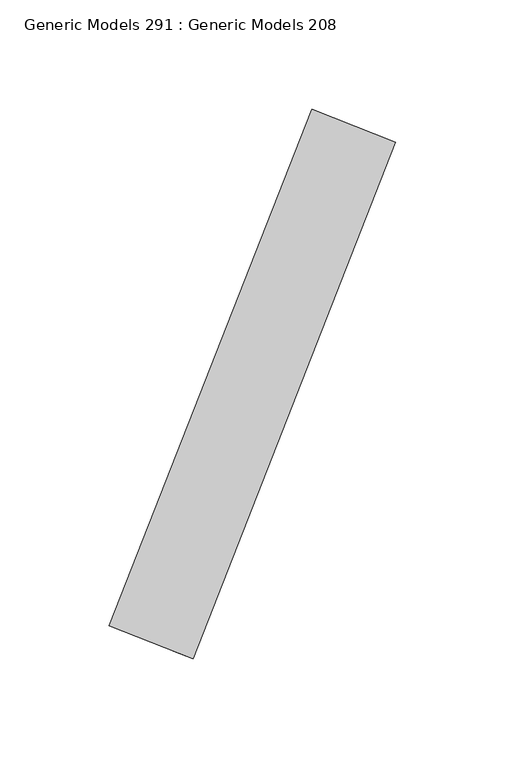
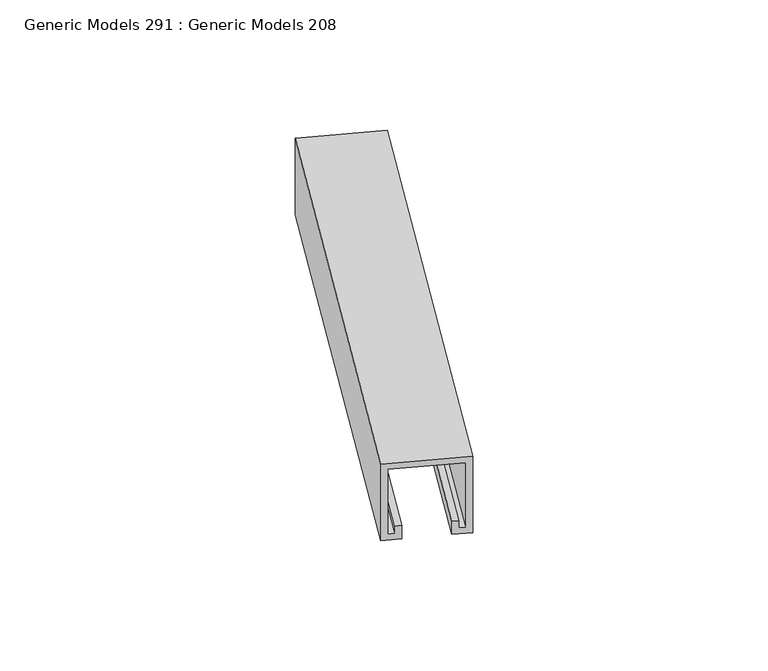
"""IFC4 building model written with IfcOpenShell, lengths in millimetres: proxy geometry, Generic Models 291 : Generic Models 208."""

from ifc_helpers import new_model, si_unit, frame, origin, place, context, project, spatial, polyline, outline, extrude, source, transform, mapped, element, save


def generic_models_291_generic_models_208_e54af5be(model_context):
    return source(origin(), model_context, "Body", "SweptSolid", [
        extrude(outline(polyline([(-3.175, 0.0), (-3.175, 34.9250001), (-38.1, 34.9250001), (-38.1, 31.7500001), (-34.13125, 31.7500001), (-34.13125, 28.575), (-41.275, 28.575), (-41.275, 38.1000001), (0.0, 38.1000001), (0.0, -3.175), (-41.275, -3.175), (-41.275, 6.35), (-34.13125, 6.35), (-34.13125, 3.1750001), (-38.1, 3.1750001), (-38.1, 0.0), (-3.175, 0.0)])), frame((189.4518594, -22488.7252981, 1035.05), z_axis=(0.36539272668216666, 0.9308534553235388, 0.0), x_axis=(0.0, 0.0, 1.0)), (0.0, 0.0, 1.0), 254.0),
    ])


if __name__ == "__main__":
    model = new_model("IFC4")
    model_context = context("Model", 3, world=origin())
    ifc_project = project(units=[si_unit("LENGTHUNIT", "METRE", prefix="MILLI")], contexts=[model_context])
    site = spatial("IfcSite", under=ifc_project)
    building = spatial("IfcBuilding", under=site)
    placement = place(None, origin())
    generic_models_291_generic_models_208_shape = generic_models_291_generic_models_208_e54af5be(model_context)
    element("IfcBuildingElementProxy", 1, Name="Generic Models 291 : Generic Models 208", ObjectType="Generic Models 291 : Generic Models 208", at=placement, inside=building, context=model_context, shape_type="MappedRepresentation", body=[
        mapped(generic_models_291_generic_models_208_shape, transform((0.0, 0.0, 0.0), x_axis=(1.0, 0.0, 0.0), y_axis=(0.0, 1.0, 0.0), z_axis=(0.0, 0.0, 1.0))),
    ])
    save(model, "model.ifc")

# Revit data of these elements
# Element 1 (IfcBuildingElementProxy, "Generic Models 291 : Generic Models 208")
#   Materials on its faces: "UNISTRUT P1000, 1 5/8\" X 1 5/8\", CHANNEL OR ALUM. CHANNEL"
# Materials
#   "UNISTRUT P1000, 1 5/8\" X 1 5/8\", CHANNEL OR ALUM. CHANNEL": class "Metal", colour RGB 244 244 244, transparency 0, Description = "Aluminum 6061", Cost = 0
